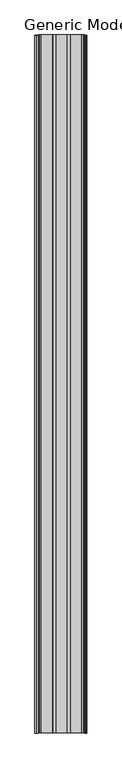
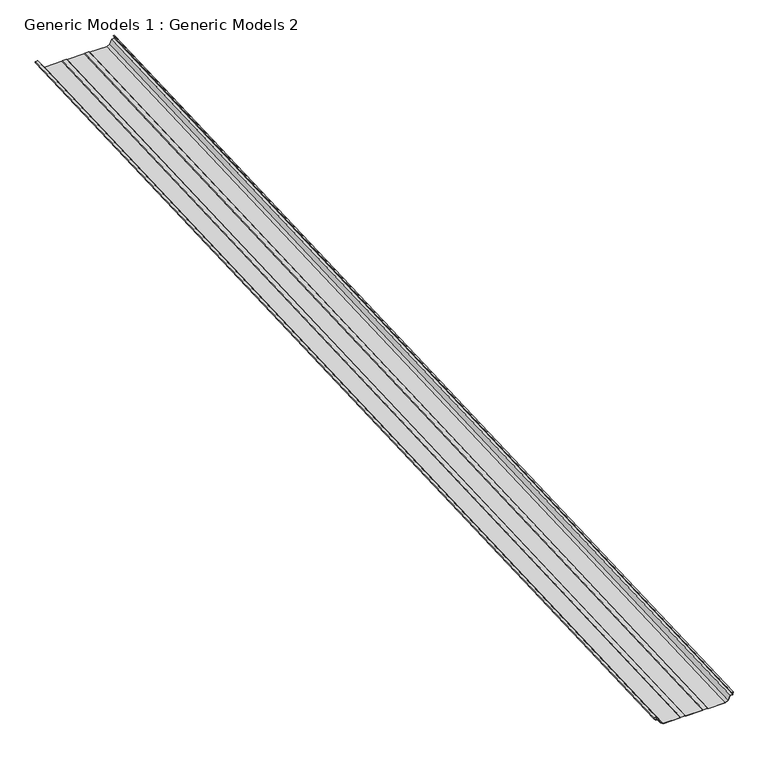
"""IFC4 building model written with IfcOpenShell, lengths in millimetres: proxy geometry, Generic Models 1 : Generic Models 2."""

from ifc_helpers import new_model, si_unit, frame, origin, place, context, project, spatial, polyline, outline, extrude, source, transform, mapped, element, save


def generic_models_1_generic_models_2_ba676d98(model_context):
    return source(origin(), model_context, "Body", "SweptSolid", [
        extrude(outline(polyline([(-1.5875, 0.0), (0.0, 0.0), (0.0, -16.2527441), (24.0067186, -12.4831292), (14.9619735, 23.6899918), (43.7640409, 30.8299277), (52.0975205, 89.5519075), (79.1719273, 115.6258501), (273.2212505, 163.730026), (278.7617463, 157.9769958), (327.4189624, 170.0389563), (329.6308632, 177.7137797), (524.274866, 225.9653747), (529.8153618, 220.2123444), (578.4725779, 232.274305), (580.6844787, 239.9491283), (776.3953745, 288.4652025), (813.7581754, 278.4253413), (848.5981807, 230.3385881), (877.3735955, 237.4719168), (886.4950159, 201.3639398), (870.8785325, 197.492666), (870.4965582, 199.0335268), (884.5653238, 202.5211266), (876.2215358, 235.5507741), (847.9408601, 228.5400895), (812.8027773, 277.0382539), (776.3793775, 286.8256861), (581.9560718, 238.6288011), (579.7441709, 230.9539778), (529.3077037, 218.4509468), (523.7672079, 224.2039771), (330.9024563, 176.3934525), (328.6905555, 168.7186291), (278.2540882, 156.2155982), (272.7135923, 161.9686284), (79.9667571, 114.1873348), (53.5924659, 88.7876368), (45.1853406, 29.5467121), (16.8879223, 22.5318771), (25.9678946, -13.7821306), (-1.5875, -18.1089705), (-1.5875, 0.0)])), frame((600943.0049991, -580698.7624569, 3927.2442762), z_axis=(0.0, 0.9991330730923522, 0.041630544712176844), x_axis=(0.9706209647694318, -0.010016878541707262, 0.24040508500100027)), (0.0, 0.0, 1.0), 12363.5881655),
    ])


if __name__ == "__main__":
    model = new_model("IFC4")
    model_context = context("Model", 3, world=origin())
    ifc_project = project(units=[si_unit("LENGTHUNIT", "METRE", prefix="MILLI")], contexts=[model_context])
    site = spatial("IfcSite", under=ifc_project)
    building = spatial("IfcBuilding", under=site)
    placement = place(None, origin())
    generic_models_1_generic_models_2_shape = generic_models_1_generic_models_2_ba676d98(model_context)
    element("IfcBuildingElementProxy", 1, Name="Generic Models 1 : Generic Models 2", ObjectType="Generic Models 1 : Generic Models 2", at=placement, inside=building, context=model_context, shape_type="MappedRepresentation", body=[
        mapped(generic_models_1_generic_models_2_shape, transform((0.0, 0.0, 0.0), x_axis=(1.0, 0.0, 0.0), y_axis=(0.0, 1.0, 0.0), z_axis=(0.0, 0.0, 1.0))),
    ])
    save(model, "model.ifc")
